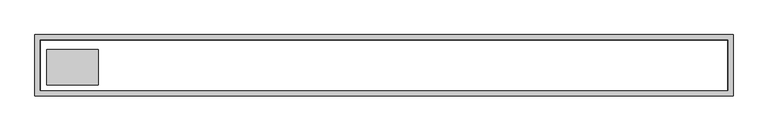
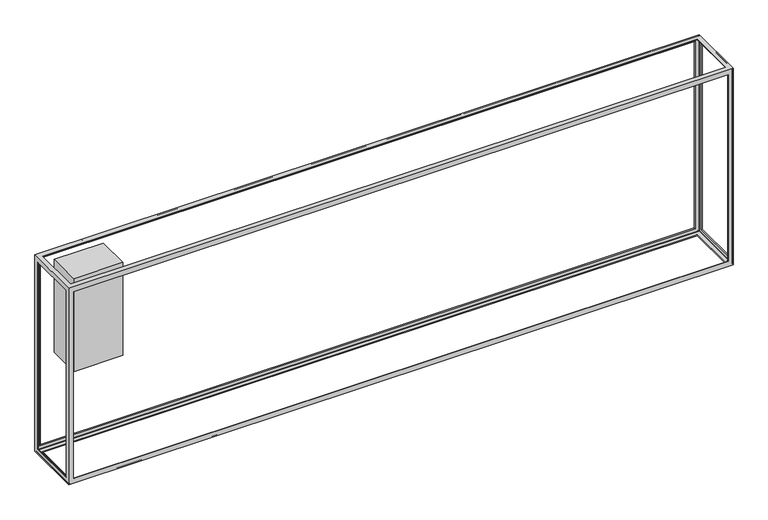
"""IFC4 building model written with IfcOpenShell, lengths in millimetres: beam geometry, Plumbing Bulkhead : EX. BULKHEAD 1."""

from ifc_helpers import new_model, si_unit, frame, origin, place, context, project, spatial, polyline, ellipse_curve, outline, extrude, source, transform, mapped, element, save
from ifc_brep_helpers import plane_surface, cylinder_surface, revolved_surface, advanced_brep


def beam_ed15209c(model_context):
    return source(origin(), model_context, "Body", "SolidModel", [
        extrude(outline(polyline([(379.0365927, 279.4), (379.0365927, 66.5145898), (70.4236299, 66.5145898), (70.4236299, 279.4), (379.0365927, 279.4)])), frame((0.0, 0.0, 688.452765), z_axis=(0.0, 0.0, 1.0), x_axis=(1.0, 0.0, 0.0)), (0.0, 0.0, 1.0), 619.647235),
        advanced_brep(
        [(0.0, 0.0, 1308.1), (0.0, 368.3, 1308.1), (0.0, 368.3, 0.0), (0.0, 0.0, 0.0), (0.0, 31.75, 1276.35), (0.0, 31.75, 31.75), (0.0, 336.55, 31.75), (0.0, 336.55, 1276.35), (4191.0, 368.3, 1308.1), (4191.0, 368.3, 0.0), (4159.25, 368.3, 31.75), (4159.25, 368.3, 1276.35), (31.75, 368.3, 1276.35), (31.75, 368.3, 31.75), (4191.0, 0.0, 0.0), (4159.25, 336.55, 0.0), (31.75, 336.55, 0.0), (31.75, 31.75, 0.0), (4159.25, 31.75, 0.0), (4191.0, 0.0, 1308.1), (4159.25, 0.0, 1276.35), (4159.25, 0.0, 31.75), (31.75, 0.0, 31.75), (31.75, 0.0, 1276.35), (3.175, 28.575, 1279.525), (3.175, 28.575, 28.575), (3.175, 339.725, 28.575), (3.175, 339.725, 1279.525), (4191.0, 336.55, 31.75), (4187.825, 339.725, 28.575), (4187.825, 28.575, 28.575), (4191.0, 31.75, 31.75), (4191.0, 31.75, 1276.35), (4191.0, 336.55, 1276.35), (4187.825, 28.575, 1279.525), (4187.825, 339.725, 1279.525), (4162.425, 339.725, 3.175), (28.575, 339.725, 3.175), (28.575, 28.575, 3.175), (4162.425, 28.575, 3.175), (4186.2375, 4.7625, 3.175), (4186.2375, 363.5375, 3.175), (4.7625, 363.5375, 3.175), (4.7625, 4.7625, 3.175), (4187.360032, 364.660032, 3.639968), (4187.360032, 3.639968, 3.639968), (4187.825, 4.7625, 4.7625), (4187.825, 363.5375, 4.7625), (4186.2375, 365.125, 4.7625), (4.7625, 365.125, 4.7625), (3.639968, 364.660032, 3.639968), (3.175, 363.5375, 4.7625), (3.175, 4.7625, 4.7625), (3.639968, 3.639968, 3.639968), (4.7625, 3.175, 4.7625), (4186.2375, 3.175, 4.7625), (4186.2375, 365.125, 1303.3375), (4.7625, 365.125, 1303.3375), (4162.425, 365.125, 1279.525), (4162.425, 365.125, 28.575), (28.575, 365.125, 28.575), (28.575, 365.125, 1279.525), (3.639968, 364.660032, 1304.460032), (3.175, 363.5375, 1303.3375), (4187.825, 363.5375, 1303.3375), (4187.360032, 364.660032, 1304.460032), (4187.825, 4.7625, 1303.3375), (4186.2375, 3.175, 1303.3375), (4187.360032, 3.639968, 1304.460032), (3.175, 4.7625, 1303.3375), (4.7625, 3.175, 1303.3375), (3.639968, 3.639968, 1304.460032), (4162.425, 3.175, 1279.525), (4162.425, 3.175, 28.575), (28.575, 3.175, 28.575), (28.575, 3.175, 1279.525), (31.75, 31.75, 1308.1), (31.75, 336.55, 1308.1), (4159.25, 336.55, 1308.1), (4159.25, 31.75, 1308.1), (28.575, 339.725, 1304.925), (4162.425, 339.725, 1304.925), (4.7625, 4.7625, 1304.925), (4.7625, 363.5375, 1304.925), (4186.2375, 363.5375, 1304.925), (4186.2375, 4.7625, 1304.925), (28.575, 28.575, 1304.925), (4162.425, 28.575, 1304.925)],
        [
            (0, 1),
            (1, 2),
            (2, 3),
            (3, 0),
            (4, 5),
            (5, 6),
            (6, 7),
            (7, 4),
            (8, 9),
            (9, 2),
            (1, 8),
            (10, 11),
            (11, 12),
            (12, 13),
            (13, 10),
            (9, 14),
            (14, 3),
            (15, 16),
            (16, 17),
            (17, 18),
            (18, 15),
            (14, 19),
            (19, 0),
            (20, 21),
            (21, 22),
            (22, 23),
            (23, 20),
            (4, 24, ellipse_curve(frame((0.0, 28.575, 1279.525), z_axis=(0.0, -0.7071067811865464, -0.7071067811865487), x_axis=(0.0, 0.7071067811865487, -0.7071067811865464)), 4.4901281, 3.175)),
            (24, 25),
            (25, 5, ellipse_curve(frame((0.0, 28.575, 28.575), z_axis=(0.0, -0.7071067811865499, 0.7071067811865451), x_axis=(0.0, -0.7071067811865451, -0.7071067811865498)), 4.4901281, 3.175)),
            (25, 26),
            (26, 6, ellipse_curve(frame((0.0, 339.725, 28.575), z_axis=(0.0, -0.707106781186545, -0.70710678118655), x_axis=(0.0, -0.7071067811865501, 0.7071067811865449)), 4.4901281, 3.175)),
            (27, 7, ellipse_curve(frame((0.0, 339.725, 1279.525), z_axis=(0.0, 0.7071067811865487, -0.7071067811865464), x_axis=(0.0, -0.7071067811865465, -0.7071067811865487)), 4.4901281, 3.175)),
            (26, 27),
            (28, 29, ellipse_curve(frame((4191.0, 339.725, 28.575), z_axis=(0.0, -0.7071067811865429, -0.7071067811865522), x_axis=(0.0, -0.7071067811865521, 0.707106781186543)), 4.4901281, 3.175)),
            (29, 30),
            (30, 31, ellipse_curve(frame((4191.0, 28.575, 28.575), z_axis=(0.0, 0.7071067811865499, -0.7071067811865451), x_axis=(0.0, -0.7071067811865451, -0.70710678118655)), 4.4901281, 3.175)),
            (31, 28),
            (8, 19),
            (31, 32),
            (32, 33),
            (33, 28),
            (30, 34),
            (34, 32, ellipse_curve(frame((4191.0, 28.575, 1279.525), z_axis=(0.0, -0.7071067811865464, -0.7071067811865487), x_axis=(0.0, 0.7071067811865487, -0.7071067811865464)), 4.4901281, 3.175)),
            (33, 35, ellipse_curve(frame((4191.0, 339.725, 1279.525), z_axis=(0.0, 0.7071067811865509, -0.7071067811865441), x_axis=(0.0, -0.707106781186544, -0.7071067811865509)), 4.4901281, 3.175)),
            (35, 29),
            (15, 36, ellipse_curve(frame((4162.425, 339.725, 0.0), z_axis=(-0.7071067811865475, 0.7071067811865475, 0.0), x_axis=(-0.7071067811865476, -0.7071067811865474, 0.0)), 4.4901281, 3.175)),
            (36, 37),
            (37, 16, ellipse_curve(frame((28.575, 339.725, 0.0), z_axis=(0.7071067811865454, 0.7071067811865498, 0.0), x_axis=(-0.7071067811865497, 0.7071067811865454, 0.0)), 4.4901281, 3.175)),
            (37, 38),
            (38, 17, ellipse_curve(frame((28.575, 28.575, 0.0), z_axis=(-0.7071067811865498, 0.7071067811865452, 0.0), x_axis=(-0.7071067811865451, -0.7071067811865498, 0.0)), 4.4901281, 3.175)),
            (39, 18, ellipse_curve(frame((4162.425, 28.575, 0.0), z_axis=(-0.7071067811865475, -0.7071067811865475, 0.0), x_axis=(-0.7071067811865476, 0.7071067811865474, 0.0)), 4.4901281, 3.175)),
            (38, 39),
            (39, 36),
            (40, 41),
            (41, 42),
            (42, 43),
            (43, 40),
            (44, 41, ellipse_curve(frame((4186.2375, 363.5375, 4.7625), z_axis=(-0.7071067811865475, 0.7071067811865475, 0.0), x_axis=(0.7071067811865474, 0.7071067811865476, 0.0)), 2.245064, 1.5875)),
            (40, 45, ellipse_curve(frame((4186.2375, 4.7625, 4.7625), z_axis=(-0.7071067811865475, -0.7071067811865475, 0.0), x_axis=(-0.7071067811865474, 0.7071067811865476, 0.0)), 2.245064, 1.5875)),
            (45, 46, ellipse_curve(frame((4186.2375, 4.7625, 4.7625), z_axis=(0.0, -0.7071067811865499, 0.7071067811865451), x_axis=(0.0, 0.7071067811865451, 0.70710678118655)), 2.245064, 1.5875)),
            (46, 47),
            (47, 44, ellipse_curve(frame((4186.2375, 363.5375, 4.7625), z_axis=(0.0, 0.7071067811865429, 0.7071067811865522), x_axis=(0.0, 0.7071067811865521, -0.707106781186543)), 2.245064, 1.5875)),
            (48, 49),
            (49, 50, ellipse_curve(frame((4.7625, 363.5375, 4.7625), z_axis=(-0.7071067811865439, 0.0, 0.7071067811865511), x_axis=(0.7071067811865511, 0.0, 0.7071067811865438)), 2.245064, 1.5875)),
            (50, 42, ellipse_curve(frame((4.7625, 363.5375, 4.7625), z_axis=(-0.7071067811865454, -0.7071067811865498, 0.0), x_axis=(0.7071067811865497, -0.7071067811865454, 0.0)), 2.245064, 1.5875)),
            (44, 48, ellipse_curve(frame((4186.2375, 363.5375, 4.7625), z_axis=(0.7071067811865475, 0.0, 0.7071067811865476), x_axis=(0.7071067811865475, 0.0, -0.7071067811865475)), 2.245064, 1.5875)),
            (51, 52),
            (52, 53, ellipse_curve(frame((4.7625, 4.7625, 4.7625), z_axis=(0.0, -0.7071067811865499, 0.7071067811865451), x_axis=(0.0, 0.7071067811865451, 0.70710678118655)), 2.245064, 1.5875)),
            (53, 43, ellipse_curve(frame((4.7625, 4.7625, 4.7625), z_axis=(0.7071067811865498, -0.7071067811865452, 0.0), x_axis=(0.7071067811865451, 0.7071067811865498, 0.0)), 2.245064, 1.5875)),
            (50, 51, ellipse_curve(frame((4.7625, 363.5375, 4.7625), z_axis=(0.0, 0.707106781186545, 0.70710678118655), x_axis=(0.0, 0.7071067811865501, -0.7071067811865449)), 2.245064, 1.5875)),
            (53, 54, ellipse_curve(frame((4.7625, 4.7625, 4.7625), z_axis=(-0.7071067811865439, 0.0, 0.7071067811865511), x_axis=(0.7071067811865511, 0.0, 0.7071067811865438)), 2.245064, 1.5875)),
            (54, 55),
            (55, 45, ellipse_curve(frame((4186.2375, 4.7625, 4.7625), z_axis=(0.7071067811865475, 0.0, 0.7071067811865476), x_axis=(0.7071067811865475, 0.0, -0.7071067811865475)), 2.245064, 1.5875)),
            (48, 56),
            (56, 57),
            (57, 49),
            (58, 59),
            (59, 60),
            (60, 61),
            (61, 58),
            (57, 62, ellipse_curve(frame((4.7625, 363.5375, 1303.3375), z_axis=(0.7071067811865511, 0.0, 0.7071067811865439), x_axis=(-0.7071067811865438, 0.0, 0.7071067811865511)), 2.245064, 1.5875)),
            (62, 63, ellipse_curve(frame((4.7625, 363.5375, 1303.3375), z_axis=(0.0, -0.7071067811865487, 0.7071067811865464), x_axis=(0.0, 0.7071067811865465, 0.7071067811865487)), 2.245064, 1.5875)),
            (63, 51),
            (47, 64),
            (64, 65, ellipse_curve(frame((4186.2375, 363.5375, 1303.3375), z_axis=(0.0, -0.7071067811865509, 0.7071067811865441), x_axis=(0.0, 0.707106781186544, 0.7071067811865509)), 2.245064, 1.5875)),
            (65, 56, ellipse_curve(frame((4186.2375, 363.5375, 1303.3375), z_axis=(-0.7071067811865475, 0.0, 0.7071067811865475), x_axis=(0.7071067811865474, 0.0, 0.7071067811865476)), 2.245064, 1.5875)),
            (10, 59, ellipse_curve(frame((4162.425, 368.3, 28.575), z_axis=(0.7071067811865475, 0.0, 0.7071067811865476), x_axis=(0.7071067811865476, 0.0, -0.7071067811865475)), 4.4901281, 3.175)),
            (58, 11, ellipse_curve(frame((4162.425, 368.3, 1279.525), z_axis=(0.7071067811865475, 0.0, -0.7071067811865475), x_axis=(-0.7071067811865474, 0.0, -0.7071067811865476)), 4.4901281, 3.175)),
            (13, 60, ellipse_curve(frame((28.575, 368.3, 28.575), z_axis=(0.7071067811865439, 0.0, -0.7071067811865511), x_axis=(-0.7071067811865511, 0.0, -0.7071067811865438)), 4.4901281, 3.175)),
            (12, 61, ellipse_curve(frame((28.575, 368.3, 1279.525), z_axis=(-0.7071067811865511, 0.0, -0.7071067811865439), x_axis=(0.7071067811865438, 0.0, -0.7071067811865511)), 4.4901281, 3.175)),
            (46, 66),
            (66, 64),
            (35, 34),
            (55, 67),
            (67, 68, ellipse_curve(frame((4186.2375, 4.7625, 1303.3375), z_axis=(-0.7071067811865475, 0.0, 0.7071067811865475), x_axis=(0.7071067811865474, 0.0, 0.7071067811865476)), 2.245064, 1.5875)),
            (68, 66, ellipse_curve(frame((4186.2375, 4.7625, 1303.3375), z_axis=(0.0, 0.7071067811865464, 0.7071067811865487), x_axis=(0.0, -0.7071067811865487, 0.7071067811865464)), 2.245064, 1.5875)),
            (63, 69),
            (69, 52),
            (24, 27),
            (70, 54),
            (69, 71, ellipse_curve(frame((4.7625, 4.7625, 1303.3375), z_axis=(0.0, 0.7071067811865464, 0.7071067811865487), x_axis=(0.0, -0.7071067811865487, 0.7071067811865464)), 2.245064, 1.5875)),
            (71, 70, ellipse_curve(frame((4.7625, 4.7625, 1303.3375), z_axis=(0.7071067811865511, 0.0, 0.7071067811865439), x_axis=(-0.7071067811865438, 0.0, 0.7071067811865511)), 2.245064, 1.5875)),
            (72, 73),
            (73, 21, ellipse_curve(frame((4162.425, 0.0, 28.575), z_axis=(0.7071067811865475, 0.0, 0.7071067811865476), x_axis=(0.7071067811865476, 0.0, -0.7071067811865475)), 4.4901281, 3.175)),
            (20, 72, ellipse_curve(frame((4162.425, 0.0, 1279.525), z_axis=(0.7071067811865475, 0.0, -0.7071067811865475), x_axis=(-0.7071067811865474, 0.0, -0.7071067811865476)), 4.4901281, 3.175)),
            (73, 74),
            (74, 22, ellipse_curve(frame((28.575, 0.0, 28.575), z_axis=(0.7071067811865439, 0.0, -0.7071067811865511), x_axis=(-0.7071067811865511, 0.0, -0.7071067811865438)), 4.4901281, 3.175)),
            (74, 75),
            (75, 23, ellipse_curve(frame((28.575, 0.0, 1279.525), z_axis=(-0.7071067811865511, 0.0, -0.7071067811865439), x_axis=(0.7071067811865438, 0.0, -0.7071067811865511)), 4.4901281, 3.175)),
            (70, 67),
            (72, 75),
            (76, 77),
            (77, 78),
            (78, 79),
            (79, 76),
            (77, 80, ellipse_curve(frame((28.575, 339.725, 1308.1), z_axis=(0.707106781186548, 0.7071067811865469, 0.0), x_axis=(-0.707106781186547, 0.7071067811865478, 0.0)), 4.4901281, 3.175)),
            (80, 81),
            (81, 78, ellipse_curve(frame((4162.425, 339.725, 1308.1), z_axis=(-0.7071067811865469, 0.707106781186548, 0.0), x_axis=(-0.7071067811865481, -0.7071067811865468, 0.0)), 4.4901281, 3.175)),
            (82, 83),
            (83, 84),
            (84, 85),
            (85, 82),
            (80, 86),
            (86, 87),
            (87, 81),
            (65, 84, ellipse_curve(frame((4186.2375, 363.5375, 1303.3375), z_axis=(0.7071067811865469, -0.707106781186548, 0.0), x_axis=(0.7071067811865481, 0.7071067811865468, 0.0)), 2.245064, 1.5875)),
            (83, 62, ellipse_curve(frame((4.7625, 363.5375, 1303.3375), z_axis=(-0.707106781186548, -0.7071067811865469, 0.0), x_axis=(0.707106781186547, -0.7071067811865478, 0.0)), 2.245064, 1.5875)),
            (86, 76, ellipse_curve(frame((28.575, 28.575, 1308.1), z_axis=(0.7071067811865469, -0.707106781186548, 0.0), x_axis=(-0.7071067811865481, -0.7071067811865468, 0.0)), 4.4901281, 3.175)),
            (79, 87, ellipse_curve(frame((4162.425, 28.575, 1308.1), z_axis=(-0.707106781186548, -0.7071067811865469, 0.0), x_axis=(-0.707106781186547, 0.7071067811865478, 0.0)), 4.4901281, 3.175)),
            (71, 82, ellipse_curve(frame((4.7625, 4.7625, 1303.3375), z_axis=(-0.7071067811865469, 0.707106781186548, 0.0), x_axis=(0.7071067811865481, 0.7071067811865468, 0.0)), 2.245064, 1.5875)),
            (85, 68, ellipse_curve(frame((4186.2375, 4.7625, 1303.3375), z_axis=(0.707106781186548, 0.7071067811865469, 0.0), x_axis=(0.707106781186547, -0.7071067811865478, 0.0)), 2.245064, 1.5875)),
        ],
        [
            plane_surface(frame((0.0, 368.3, 0.0), z_axis=(-1.0, 0.0, 0.0), x_axis=(0.0, 0.0, 1.0))),
            plane_surface(frame((0.0, 368.3, 31.75), z_axis=(0.0, 1.0, 0.0), x_axis=(1.0, 0.0, 0.0))),
            plane_surface(frame((0.0, 368.3, 0.0), z_axis=(0.0, 0.0, -1.0), x_axis=(1.0, 0.0, 0.0))),
            plane_surface(frame((4191.0, 0.0, 0.0), z_axis=(0.0, -1.0, 0.0), x_axis=(0.0, 0.0, 1.0))),
            cylinder_surface(frame((0.0, 28.575, 0.0), z_axis=(0.0, 0.0, -1.0), x_axis=(0.0, 1.0, 0.0)), 3.175),
            cylinder_surface(frame((0.0, 0.0, 28.575), z_axis=(0.0, -1.0, 0.0), x_axis=(1.0, 0.0, 0.0)), 3.175),
            cylinder_surface(frame((0.0, 339.725, 0.0), z_axis=(0.0, 0.0, -1.0), x_axis=(0.0, -1.0, 0.0)), 3.175),
            cylinder_surface(frame((4191.0, 0.0, 28.575), z_axis=(0.0, -1.0, 0.0), x_axis=(-1.0, 0.0, 0.0)), 3.175),
            plane_surface(frame((4191.0, 368.3, 0.0), z_axis=(1.0, 0.0, 0.0), x_axis=(0.0, 0.0, 1.0))),
            cylinder_surface(frame((4191.0, 28.575, 0.0), z_axis=(0.0, 0.0, -1.0), x_axis=(0.0, 1.0, 0.0)), 3.175),
            cylinder_surface(frame((4191.0, 339.725, 0.0), z_axis=(0.0, 0.0, -1.0), x_axis=(0.0, -1.0, 0.0)), 3.175),
            cylinder_surface(frame((0.0, 339.725, 0.0), z_axis=(-1.0, 0.0, 0.0), x_axis=(0.0, -1.0, 0.0)), 3.175),
            cylinder_surface(frame((28.575, 0.0, 0.0), z_axis=(0.0, -1.0, 0.0), x_axis=(1.0, 0.0, 0.0)), 3.175),
            cylinder_surface(frame((0.0, 28.575, 0.0), z_axis=(-1.0, 0.0, 0.0), x_axis=(0.0, 1.0, 0.0)), 3.175),
            cylinder_surface(frame((4162.425, 0.0, 0.0), z_axis=(0.0, -1.0, 0.0), x_axis=(-1.0, 0.0, 0.0)), 3.175),
            plane_surface(frame((0.0, 339.725, 3.175), z_axis=(0.0, 0.0, 1.0), x_axis=(1.0, 0.0, 0.0))),
            revolved_surface(polyline([(4184.650000000001, 365.1249999785978, 4.7625), (4184.650000000001, 3.1750000214022047, 4.7625)]), (4186.2375, 0.0, 4.7625), (0.0, 1.0, 0.0)),
            revolved_surface(polyline([(4187.824999978598, 361.95000000000005, 4.7625), (3.175000021402197, 361.95000000000005, 4.7625)]), (0.0, 363.5375, 4.7625), (1.0, 0.0, 0.0)),
            revolved_surface(polyline([(6.35, 365.1249999785978, 4.7625), (6.35, 3.1750000214022, 4.7625)]), (4.7625, 0.0, 4.7625), (0.0, 1.0, 0.0)),
            revolved_surface(polyline([(4187.824999978598, 6.35, 4.7625), (3.175000021402197, 6.35, 4.7625)]), (0.0, 4.7625, 4.7625), (1.0, 0.0, 0.0)),
            plane_surface(frame((0.0, 365.125, 4.7625), z_axis=(0.0, -1.0, 0.0), x_axis=(1.0, 0.0, 0.0))),
            revolved_surface(polyline([(4.7625, 361.95000000000005, 1304.924999978598), (4.7625, 361.95000000000005, 3.1750000214022105)]), (4.7625, 363.5375, 0.0), (0.0, 0.0, 1.0)),
            revolved_surface(polyline([(4186.2375, 361.95000000000005, 1304.924999978598), (4186.2375, 361.95000000000005, 3.175000021402205)]), (4186.2375, 363.5375, 0.0), (0.0, 0.0, 1.0)),
            cylinder_surface(frame((4162.425, 368.3, 0.0), z_axis=(0.0, 0.0, -1.0), x_axis=(0.0, -1.0, 0.0)), 3.175),
            cylinder_surface(frame((0.0, 368.3, 28.575), z_axis=(-1.0, 0.0, 0.0), x_axis=(0.0, -1.0, 0.0)), 3.175),
            cylinder_surface(frame((28.575, 368.3, 0.0), z_axis=(0.0, 0.0, -1.0), x_axis=(0.0, -1.0, 0.0)), 3.175),
            plane_surface(frame((4187.825, 339.725, 0.0), z_axis=(-1.0, 0.0, 0.0), x_axis=(0.0, 0.0, 1.0))),
            revolved_surface(polyline([(4186.2375, 6.35, 1304.924999978598), (4186.2375, 6.35, 3.1750000214021994)]), (4186.2375, 4.7625, 0.0), (0.0, 0.0, 1.0)),
            plane_surface(frame((3.175, 363.5375, 0.0), z_axis=(1.0, 0.0, 0.0), x_axis=(0.0, 0.0, 1.0))),
            revolved_surface(polyline([(4.7625, 6.35, 1304.924999978598), (4.7625, 6.35, 3.1750000214021994)]), (4.7625, 4.7625, 0.0), (0.0, 0.0, 1.0)),
            cylinder_surface(frame((4162.425, 0.0, 0.0), z_axis=(0.0, 0.0, -1.0), x_axis=(0.0, 1.0, 0.0)), 3.175),
            cylinder_surface(frame((0.0, 0.0, 28.575), z_axis=(-1.0, 0.0, 0.0), x_axis=(0.0, 1.0, 0.0)), 3.175),
            cylinder_surface(frame((28.575, 0.0, 0.0), z_axis=(0.0, 0.0, -1.0), x_axis=(0.0, 1.0, 0.0)), 3.175),
            plane_surface(frame((0.0, 3.175, 1303.3375), z_axis=(0.0, 1.0, 0.0), x_axis=(1.0, 0.0, 0.0))),
            plane_surface(frame((4191.0, 368.3, 1308.1), z_axis=(0.0, 0.0, 1.0), x_axis=(1.0, 0.0, 0.0))),
            cylinder_surface(frame((0.0, 339.725, 1308.1), z_axis=(-1.0, 0.0, 0.0), x_axis=(0.0, -1.0, 0.0)), 3.175),
            plane_surface(frame((0.0, 363.5375, 1304.925), z_axis=(0.0, 0.0, -1.0), x_axis=(1.0, 0.0, 0.0))),
            revolved_surface(polyline([(4187.824999978598, 361.95000000000005, 1303.3375), (3.175000021402206, 361.95000000000005, 1303.3375)]), (0.0, 363.5375, 1303.3375), (1.0, 0.0, 0.0)),
            cylinder_surface(frame((0.0, 368.3, 1279.525), z_axis=(-1.0, 0.0, 0.0), x_axis=(0.0, -1.0, 0.0)), 3.175),
            cylinder_surface(frame((0.0, 28.575, 1308.1), z_axis=(-1.0, 0.0, 0.0), x_axis=(0.0, 1.0, 0.0)), 3.175),
            revolved_surface(polyline([(4187.824999978598, 6.35, 1303.3375), (3.1750000214022034, 6.35, 1303.3375)]), (0.0, 4.7625, 1303.3375), (1.0, 0.0, 0.0)),
            cylinder_surface(frame((0.0, 0.0, 1279.525), z_axis=(-1.0, 0.0, 0.0), x_axis=(0.0, 1.0, 0.0)), 3.175),
            cylinder_surface(frame((28.575, 0.0, 1308.1), z_axis=(0.0, -1.0, 0.0), x_axis=(1.0, 0.0, 0.0)), 3.175),
            revolved_surface(polyline([(6.35, 365.1249999785978, 1303.3375), (6.35, 3.1750000214022025, 1303.3375)]), (4.7625, 0.0, 1303.3375), (0.0, 1.0, 0.0)),
            cylinder_surface(frame((0.0, 0.0, 1279.525), z_axis=(0.0, -1.0, 0.0), x_axis=(1.0, 0.0, 0.0)), 3.175),
            cylinder_surface(frame((4162.425, 0.0, 1308.1), z_axis=(0.0, -1.0, 0.0), x_axis=(-1.0, 0.0, 0.0)), 3.175),
            revolved_surface(polyline([(4184.650000000001, 365.1249999785978, 1303.3375), (4184.650000000001, 3.1750000214022025, 1303.3375)]), (4186.2375, 0.0, 1303.3375), (0.0, 1.0, 0.0)),
            cylinder_surface(frame((4191.0, 0.0, 1279.525), z_axis=(0.0, -1.0, 0.0), x_axis=(-1.0, 0.0, 0.0)), 3.175),
        ],
        [
            (0, [[1, 2, 3, 4], [5, 6, 7, 8]]),
            (1, [[9, 10, -2, 11], [12, 13, 14, 15]]),
            (2, [[-3, -10, 16, 17], [18, 19, 20, 21]]),
            (3, [[-17, 22, 23, -4], [24, 25, 26, 27]]),
            (4, [[28, 29, 30, -5]]),
            (5, [[31, 32, -6, -30]]),
            (6, [[33, -7, -32, 34]]),
            (7, [[35, 36, 37, 38]]),
            (8, [[-16, -9, 39, -22], [-38, 40, 41, 42]]),
            (9, [[-37, 43, 44, -40]]),
            (10, [[-35, -42, 45, 46]]),
            (11, [[47, 48, 49, -18]]),
            (12, [[-19, -49, 50, 51]]),
            (13, [[52, -20, -51, 53]]),
            (14, [[-47, -21, -52, 54]]),
            (15, [[55, 56, 57, 58], [-54, -53, -50, -48]]),
            (16, [[59, -55, 60, 61, 62, 63]]),
            (17, [[64, 65, 66, -56, -59, 67]]),
            (18, [[68, 69, 70, -57, -66, 71]]),
            (19, [[-60, -58, -70, 72, 73, 74]]),
            (20, [[75, 76, 77, -64], [78, 79, 80, 81]]),
            (21, [[-77, 82, 83, 84, -71, -65]]),
            (22, [[-75, -67, -63, 85, 86, 87]]),
            (23, [[88, -78, 89, -12]]),
            (24, [[-88, -15, 90, -79]]),
            (25, [[-80, -90, -14, 91]]),
            (26, [[-62, 92, 93, -85], [-36, -46, 94, -43]]),
            (27, [[-61, -74, 95, 96, 97, -92]]),
            (28, [[98, 99, -68, -84], [100, -34, -31, -29]]),
            (29, [[101, -72, -69, -99, 102, 103]]),
            (30, [[104, 105, -24, 106]]),
            (31, [[-105, 107, 108, -25]]),
            (32, [[109, 110, -26, -108]]),
            (33, [[-95, -73, -101, 111], [-104, 112, -109, -107]]),
            (34, [[-1, -23, -39, -11], [113, 114, 115, 116]]),
            (35, [[117, 118, 119, -114]]),
            (36, [[120, 121, 122, 123], [124, 125, 126, -118]]),
            (37, [[-76, -87, 127, -121, 128, -82]]),
            (38, [[-89, -81, -91, -13]]),
            (39, [[129, -116, 130, -125]]),
            (40, [[-111, -103, 131, -123, 132, -96]]),
            (41, [[-106, -27, -110, -112]]),
            (42, [[-113, -129, -124, -117]]),
            (43, [[-128, -120, -131, -102, -98, -83]]),
            (44, [[-8, -33, -100, -28]]),
            (45, [[-126, -130, -115, -119]]),
            (46, [[-86, -93, -97, -132, -122, -127]]),
            (47, [[-41, -44, -94, -45]]),
        ],
    ),
    ])


if __name__ == "__main__":
    model = new_model("IFC4")
    model_context = context("Model", 3, world=origin())
    ifc_project = project(units=[si_unit("LENGTHUNIT", "METRE", prefix="MILLI")], contexts=[model_context])
    site = spatial("IfcSite", under=ifc_project)
    building = spatial("IfcBuilding", under=site)
    placement = place(None, origin())
    beam_shape = beam_ed15209c(model_context)
    element("IfcBeam", 1, ObjectType="Plumbing Bulkhead : EX. BULKHEAD 1", at=placement, inside=building, context=model_context, shape_type="MappedRepresentation", body=[
        mapped(beam_shape, transform((0.0, 0.0, 0.0), x_axis=(1.0, 0.0, 0.0), y_axis=(0.0, 1.0, 0.0), z_axis=(0.0, 0.0, 1.0))),
    ])
    save(model, "model.ifc")

# Revit data of these elements
# Type "Plumbing Bulkhead : EX. BULKHEAD 1"
#   Length = 13' - 9"
#   Height = 4' - 3 1/2"
#   Depth = 1' - 2 1/2"
#   Structural Material = USE EXISTING BULKHEADS IN STORAGE (MODIFY AS NECESSARY)
#   EP MATERIAL = ELECTRICAL PANEL
# Element 1 (IfcBeam, "Plumbing Bulkhead : EX. BULKHEAD 1")
#   Materials on its faces: "USE EXISTING BULKHEADS IN STORAGE (MODIFY AS NECESSARY)", "ELECTRICAL PANEL"
# Materials
#   "USE EXISTING BULKHEADS IN STORAGE (MODIFY AS NECESSARY)": class "Generic", colour RGB 120 120 120, transparency 0, Cost = 0
#   "ELECTRICAL PANEL": class "Generic", colour RGB 255 255 255, transparency 0, Cost = 0
